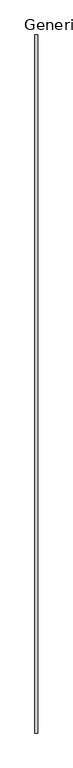
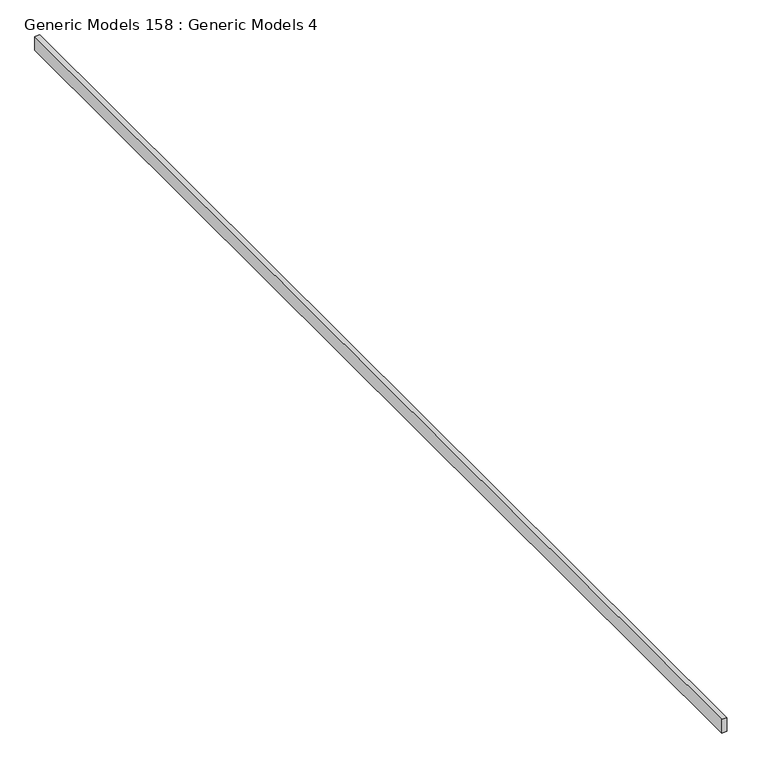
"""IFC4 building model written with IfcOpenShell, lengths in millimetres: proxy geometry, Generic Models 158 : Generic Models 4."""

from ifc_helpers import new_model, si_unit, origin, place, context, project, spatial, faceted_brep, source, transform, mapped, element, save


def generic_models_158_generic_models_4_200d1b92(model_context):
    return source(origin(), model_context, "Body", "Brep", [
        faceted_brep([(-10290.0847239, -5493.3230338, 122784.1984874), (-10290.0847239, -5493.3230338, 122631.7984874), (-10239.2847239, -5493.3230338, 122631.7984874), (-10239.2847239, -5493.3230338, 122784.1984874), (-10252.9339552, -5493.3230338, 122784.1984874), (-10290.0847239, 7054.2769662, 122784.1984874), (-10252.9339552, 7054.2769662, 122784.1984874), (-10239.2847239, 7054.2769662, 122784.1984874), (-10239.2847239, 7054.2769662, 122631.7984874), (-10290.0847239, 7054.2769662, 122631.7984874)], [[[0, 1, 2, 3, 4]], [[5, 6, 7, 8, 9]], [[1, 0, 5, 9]], [[2, 1, 9, 8]], [[3, 2, 8, 7]], [[0, 4, 3, 7, 6, 5]]]),
    ])


if __name__ == "__main__":
    model = new_model("IFC4")
    model_context = context("Model", 3, world=origin())
    ifc_project = project(units=[si_unit("LENGTHUNIT", "METRE", prefix="MILLI")], contexts=[model_context])
    site = spatial("IfcSite", under=ifc_project)
    building = spatial("IfcBuilding", under=site)
    placement = place(None, origin())
    generic_models_158_generic_models_4_shape = generic_models_158_generic_models_4_200d1b92(model_context)
    element("IfcBuildingElementProxy", 1, Name="Generic Models 158 : Generic Models 4", ObjectType="Generic Models 158 : Generic Models 4", at=placement, inside=building, context=model_context, shape_type="MappedRepresentation", body=[
        mapped(generic_models_158_generic_models_4_shape, transform((0.0, 0.0, 0.0), x_axis=(1.0, 0.0, 0.0), y_axis=(0.0, 1.0, 0.0), z_axis=(0.0, 0.0, 1.0))),
    ])
    save(model, "model.ifc")

# Revit data of these elements
# Element 1 (IfcBuildingElementProxy, "Generic Models 158 : Generic Models 4")
#   Materials on its faces: "_SPLIT FACE STONE VENEER"
# Materials
#   "_SPLIT FACE STONE VENEER": class "Generic", colour RGB 125 135 145, transparency 0, Cost = 0
